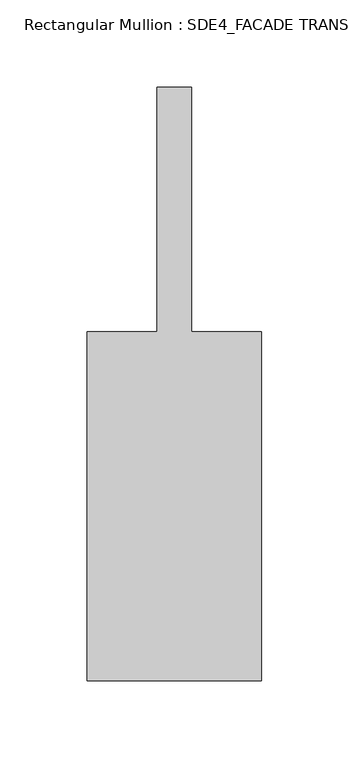
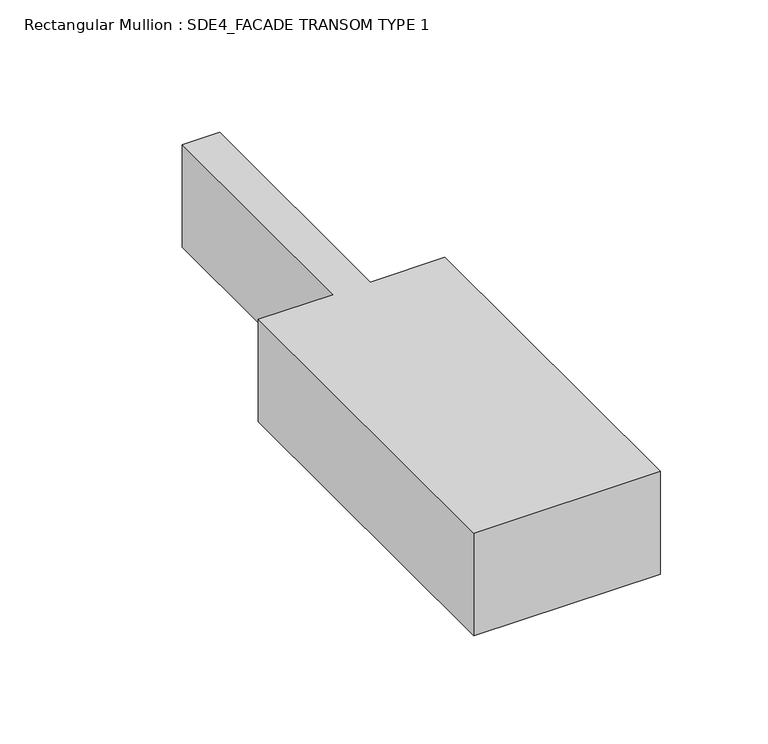
"""IFC4 building model written with IfcOpenShell, lengths in millimetres: member geometry, Rectangular Mullion : SDE4_FACADE TRANSOM TYPE 1."""

from ifc_helpers import new_model, si_unit, frame, origin, place, context, project, spatial, polyline, outline, extrude, source, transform, mapped, element, save


def rectangular_mullion_sde4_facade_transom_type_1_a58332c9(model_context):
    return source(origin(), model_context, "Body", "SweptSolid", [
        extrude(outline(polyline([(50.0, -132.5), (-50.0, -132.5), (-50.0, 67.5), (-10.0, 67.5), (-10.0, 207.5), (10.0, 207.5), (10.0, 67.5), (50.0, 67.5), (50.0, -132.5)])), frame((0.0, 0.0, -58.1984935), z_axis=(0.0, 0.0, 1.0), x_axis=(1.0, 0.0, 0.0)), (0.0, 0.0, 1.0), 58.1984935),
    ])


if __name__ == "__main__":
    model = new_model("IFC4")
    model_context = context("Model", 3, world=origin())
    ifc_project = project(units=[si_unit("LENGTHUNIT", "METRE", prefix="MILLI")], contexts=[model_context])
    site = spatial("IfcSite", under=ifc_project)
    building = spatial("IfcBuilding", under=site)
    placement = place(None, origin())
    rectangular_mullion_sde4_facade_transom_type_1_shape = rectangular_mullion_sde4_facade_transom_type_1_a58332c9(model_context)
    element("IfcMember", 1, ObjectType="Rectangular Mullion : SDE4_FACADE TRANSOM TYPE 1", at=placement, inside=building, context=model_context, shape_type="MappedRepresentation", body=[
        mapped(rectangular_mullion_sde4_facade_transom_type_1_shape, transform((0.0, 0.0, 0.0), x_axis=(1.0, 0.0, 0.0), y_axis=(0.0, 1.0, 0.0), z_axis=(0.0, 0.0, 1.0))),
    ])
    save(model, "model.ifc")

# Revit data of these elements
# Type "Rectangular Mullion : SDE4_FACADE TRANSOM TYPE 1"
#   built-in parameter 1007322 = 1.11549 (stored number, unit not read)
#   built-in parameter 1007321 = 0.164042 (stored number, unit not read)
#   built-in parameter 1007320 = 0.164042 (stored number, unit not read)
